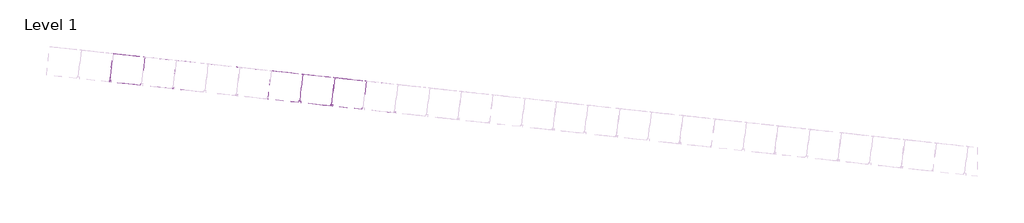
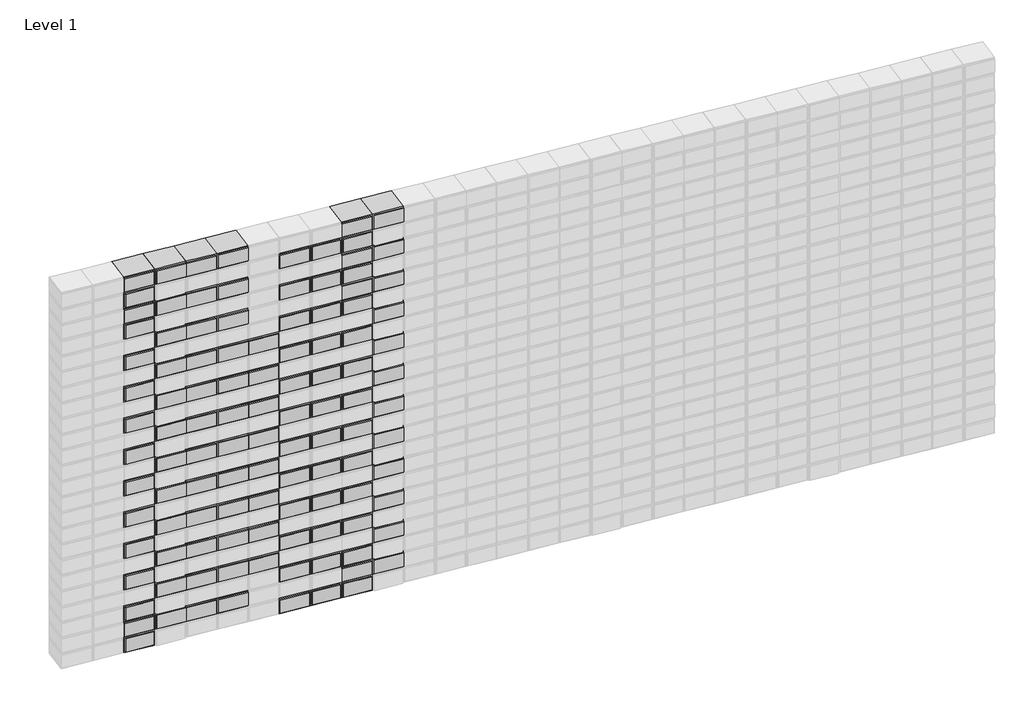
# One storey, part 12 of 18: 111 proxies.
# Revit data of these elements (continued)
# Elements 64, 65, 66, 67, 68, 69, 70, 71, 72, 73, 74, 75 (IfcBuildingElementProxy, "00_GMA_steen_versie_6 : Rood") (continued)
#   StootVoegBreedteLinks = 0 mm
#   LintVoegOnderHalf = 5 mm
#   LintVoegOnder = 10 mm
#   LintVoegBovenHalf = 5 mm
#   LintVoegBoven = 10 mm
#   Phase Created = New Construction
#   Materials on its faces: "20_voeg", "21_steen_rood"
# Elements 76, 77, 78, 79, 80, 81, 82, 83, 84, 85, 86, 87, 88, 89, 90, 91, 92, 93, 94, 95, 96, 97, 98, 99, 100, 101, 102, 103, 104, 105, 106, 107, 108, 109, 110, 111 (IfcBuildingElementProxy, "00_GMA_steen_versie_6 : Rood")
#   StootvoegLinksHalfOnder = 5 mm
#   StootvoegLinksHalfBoven = 5 mm
#   StootVoegRechtsHalfOnder = 5 mm
#   StootVoegRechtsHalfBoven = 5 mm
#   StootVoegBreedteRechts = 10 mm
#   StootVoegBreedteLinks = 10 mm
#   LintVoegOnderHalf = 5 mm
#   LintVoegOnder = 10 mm
#   LintVoegBovenHalf = 5 mm
#   LintVoegBoven = 10 mm
#   Phase Created = New Construction
#   Materials on its faces: "20_voeg", "21_steen_rood"
# Materials
#   "21_steen_geel": class "Unassigned", colour RGB 202 202 0, transparency 0, Cost = 0
#   "20_voeg": class "Concrete", colour RGB 86 86 86, transparency 0, Manufacturer = "RevitGG", URL = "www.revitgg.nl", Description = "zandcement, generiek materiaal", Cost = 0
#   "21_steen_rood": class "Unassigned", colour RGB 213 111 43, transparency 0, Cost = 0
